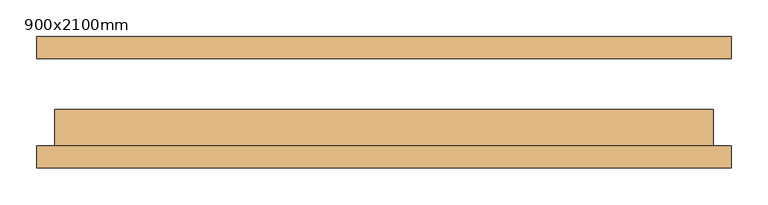
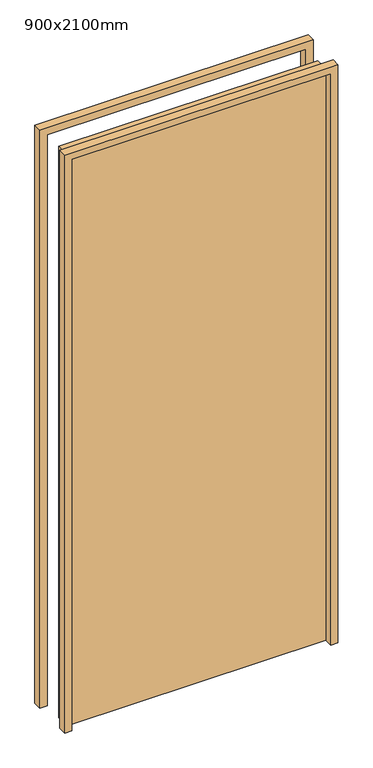
"""IFC4 building model written with IfcOpenShell, lengths in millimetres: door geometry, WWm-SingleSolid-Flush : 900x2100mm."""

from ifc_helpers import new_model, si_unit, frame, origin, origin_with_axes, place, context, project, spatial, polyline, outline, extrude, source, transform, mapped, element, save


def door_900x2100mm_017db555(model_context):
    return source(origin(), model_context, "Body", "SweptSolid", [
        extrude(outline(polyline([(2125.0, -475.0), (0.0, -475.0), (0.0, -450.0), (2100.0, -450.0), (2100.0, 450.0), (0.0, 450.0), (0.0, 475.0), (2125.0, 475.0), (2125.0, -475.0)])), frame((0.0, -90.0, 0.0), z_axis=(0.0, 1.0, 0.0), x_axis=(0.0, 0.0, 1.0)), (0.0, 0.0, 1.0), 30.0),
        extrude(outline(polyline([(2125.0, 475.0), (2125.0, -475.0), (0.0, -475.0), (0.0, -450.0), (2100.0, -450.0), (2100.0, 450.0), (0.0, 450.0), (0.0, 475.0), (2125.0, 475.0)])), frame((0.0, 60.0, 0.0), z_axis=(0.0, 1.0, 0.0), x_axis=(0.0, 0.0, 1.0)), (0.0, 0.0, 1.0), 30.0),
        extrude(outline(polyline([(450.0, -10.0), (450.0, -60.0), (-450.0, -60.0), (-450.0, -10.0), (450.0, -10.0)])), origin_with_axes(), (0.0, 0.0, 1.0), 2100.0),
    ])


if __name__ == "__main__":
    model = new_model("IFC4")
    model_context = context("Model", 3, world=origin())
    ifc_project = project(units=[si_unit("LENGTHUNIT", "METRE", prefix="MILLI")], contexts=[model_context])
    site = spatial("IfcSite", under=ifc_project)
    building = spatial("IfcBuilding", under=site)
    placement = place(None, origin())
    door_900x2100mm_shape = door_900x2100mm_017db555(model_context)
    element("IfcDoor", 1, ObjectType="WWm-SingleSolid-Flush : 900x2100mm", at=placement, inside=building, context=model_context, shape_type="MappedRepresentation", body=[
        mapped(door_900x2100mm_shape, transform((0.0, 0.0, 0.0), x_axis=(1.0, 0.0, 0.0), y_axis=(0.0, 1.0, 0.0), z_axis=(0.0, 0.0, 1.0))),
    ])
    save(model, "model.ifc")

# Revit data of these elements
# Type "WWm-SingleSolid-Flush : 900x2100mm"
#   Type Mark = "EX1-52"
#   Construction Type Id = "MDOOR"
#   Assembly Code = "C1020"
#   Analytic Construction = "Metal"
#   Thickness = 50 mm
#   Thermal Resistance (R) = 0.270117 (m²·K)/W
#   Heat Transfer Coefficient (U) = 3.7021 W/(m²·K)
#   Height = 2100 mm
#   Trim Projection Ext = 30 mm
#   Trim Projection Int = 30 mm
#   Trim Width = 25 mm
#   Width = 900 mm
#   Not 90 Degree [instance default] = no
#   90 Degree [instance default] = yes
#   Door Material = WW-EC-RGB-White
#   Frame Material = WW-EC-RGB-White
#   Visual Light Transmittance = 0
#   Solar Heat Gain Coefficient = 0
#   Function = (empty or 0)
#   Wall Closure = (empty or 0)
# Element 1 (IfcDoor, "WWm-SingleSolid-Flush : 900x2100mm")
#   Materials on its faces: "WW-EC-RGB-White"
# Materials
#   "WW-EC-RGB-White": class "Generic", colour RGB 255 255 255, transparency 0, Comments = "If region requests off-white, swith asset color to RGB 231-228-220", Description = "Generic Color", Cost = 0
